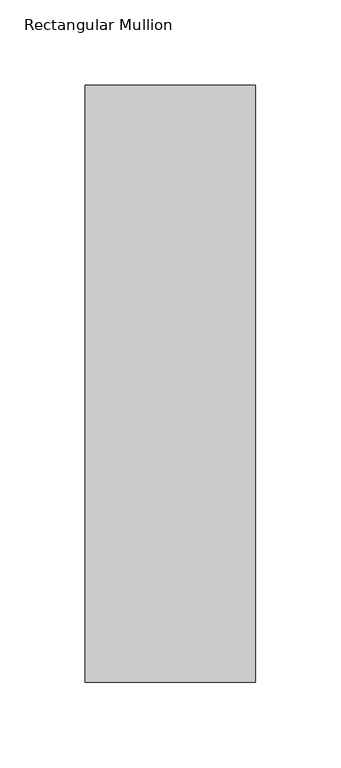
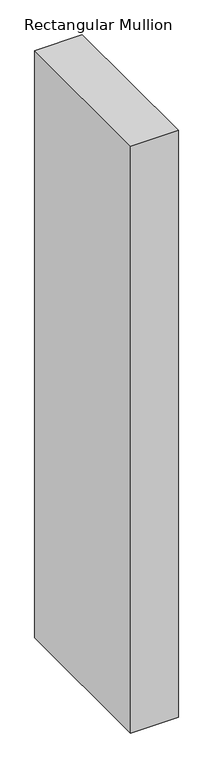
"""IFC4 building model written with IfcOpenShell, lengths in millimetres: member geometry, Rectangular Mullion : WWm-100x350-100mmOffset."""

from ifc_helpers import new_model, si_unit, frame, origin, place, context, project, spatial, polyline, outline, extrude, source, transform, mapped, element, save


def rectangular_mullion_e7d227c1(model_context):
    return source(origin(), model_context, "Body", "SweptSolid", [
        extrude(outline(polyline([(0.0, 175.0), (0.0, -175.0), (-100.0, -175.0), (-100.0, 175.0), (0.0, 175.0)])), frame((0.0, 0.0, -1305.0), z_axis=(0.0, 0.0, 1.0), x_axis=(1.0, 0.0, 0.0)), (0.0, 0.0, 1.0), 1305.0),
    ])


if __name__ == "__main__":
    model = new_model("IFC4")
    model_context = context("Model", 3, world=origin())
    ifc_project = project(units=[si_unit("LENGTHUNIT", "METRE", prefix="MILLI")], contexts=[model_context])
    site = spatial("IfcSite", under=ifc_project)
    building = spatial("IfcBuilding", under=site)
    placement = place(None, origin())
    rectangular_mullion_shape = rectangular_mullion_e7d227c1(model_context)
    element("IfcMember", 1, ObjectType="Rectangular Mullion : WWm-100x350-100mmOffset", at=placement, inside=building, context=model_context, shape_type="MappedRepresentation", body=[
        mapped(rectangular_mullion_shape, transform((0.0, 0.0, 0.0), x_axis=(1.0, 0.0, 0.0), y_axis=(0.0, 1.0, 0.0), z_axis=(0.0, 0.0, 1.0))),
    ])
    save(model, "model.ifc")

# Revit data of these elements
# Type "Rectangular Mullion : WWm-100x350-100mmOffset"
#   built-in parameter 1007304 = 1.14829 (stored number, unit not read)
#   built-in parameter 1007301 = 0.164042 (stored number, unit not read)
#   built-in parameter 1007300 = 0.164042 (stored number, unit not read)
# Element 1 (IfcMember, "Rectangular Mullion : WWm-100x350-100mmOffset")
#   Materials on its faces: "WW-EC-RGB-Mullion"
# Materials
#   "WW-EC-RGB-Mullion": class "Generic", colour RGB 255 255 255, transparency 0, Comments = "If region requests black mullions, switch asset color to RGB 25-25-25", Description = "Generic Color", Cost = 0
